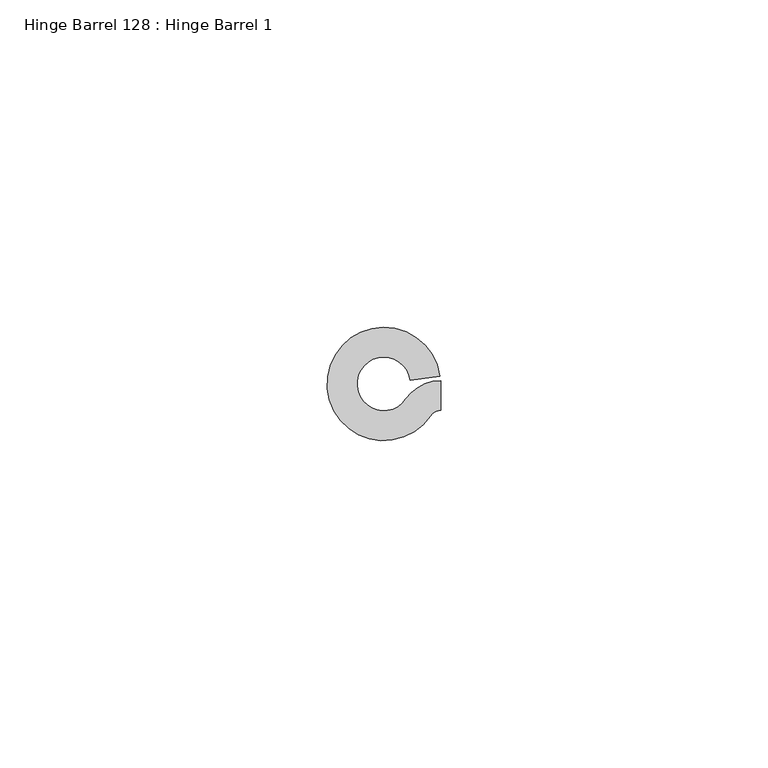
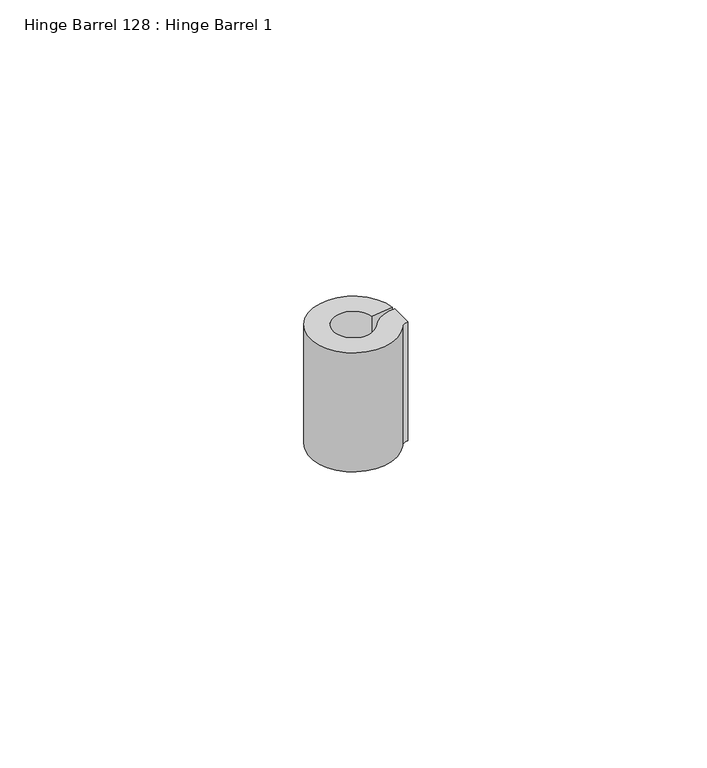
"""IFC4 building model written with IfcOpenShell, lengths in millimetres: proxy geometry, Hinge Barrel 128 : Hinge Barrel 1."""

from ifc_helpers import new_model, si_unit, point, frame, frame_2d, origin, place, context, project, spatial, polyline, circle_curve, trimmed, segment, composite_curve, outline, extrude, source, transform, mapped, element, save


def hinge_barrel_128_hinge_barrel_1_d11eb973(model_context):
    return source(origin(), model_context, "Body", "SweptSolid", [
        extrude(outline(composite_curve([segment(trimmed(circle_curve(frame_2d((587327.8245257, -536316.2443067)), 6.4044851), [point((587322.5194669, -536312.6563017))], [point((587327.8245257, -536309.8398216))], False, "CARTESIAN"), True, "CONTINUOUS"), segment(polyline([(587327.8245257, -536309.8398216), (587327.8245257, -536314.4038841)]), True, "CONTINUOUS"), segment(trimmed(circle_curve(frame_2d((587327.8245257, -536316.2443067)), 1.8404226), [point((587327.8245257, -536314.4038841))], [point((587326.3000393, -536315.2132409))], True, "CARTESIAN"), True, "CONTINUOUS"), segment(trimmed(circle_curve(frame_2d((587319.1320739, -536310.3652841)), 8.6534625), [point((587326.3000393, -536315.2132409))], [point((587327.7022899, -536309.1678654))], False, "CARTESIAN"), True, "CONTINUOUS"), segment(polyline([(587327.7022899, -536309.1678654), (587323.1821338, -536309.7994153)]), True, "CONTINUOUS"), segment(trimmed(circle_curve(frame_2d((587319.1320739, -536310.3652841)), 4.0894), [point((587323.1821338, -536309.7994153))], [point((587322.5194669, -536312.6563017))], True, "CARTESIAN"), True, "CONTINUOUS")], self_intersect=False)), frame((0.0, 0.0, 336.55), z_axis=(0.0, 0.0, 1.0), x_axis=(1.0, 0.0, 0.0)), (0.0, 0.0, 1.0), 25.4),
    ])


if __name__ == "__main__":
    model = new_model("IFC4")
    model_context = context("Model", 3, world=origin())
    ifc_project = project(units=[si_unit("LENGTHUNIT", "METRE", prefix="MILLI")], contexts=[model_context])
    site = spatial("IfcSite", under=ifc_project)
    building = spatial("IfcBuilding", under=site)
    placement = place(None, origin())
    hinge_barrel_128_hinge_barrel_1_shape = hinge_barrel_128_hinge_barrel_1_d11eb973(model_context)
    element("IfcBuildingElementProxy", 1, Name="Hinge Barrel 128 : Hinge Barrel 1", ObjectType="Hinge Barrel 128 : Hinge Barrel 1", at=placement, inside=building, context=model_context, shape_type="MappedRepresentation", body=[
        mapped(hinge_barrel_128_hinge_barrel_1_shape, transform((0.0, 0.0, 0.0), x_axis=(1.0, 0.0, 0.0), y_axis=(0.0, 1.0, 0.0), z_axis=(0.0, 0.0, 1.0))),
    ])
    save(model, "model.ifc")

# Revit data of these elements
# Element 1 (IfcBuildingElementProxy, "Hinge Barrel 128 : Hinge Barrel 1")
#   Materials on its faces: "6\"X6\" WELD-ON STL BUTT HINGE"
# Materials
#   "6\"X6\" WELD-ON STL BUTT HINGE": class "Metal", colour RGB 189 187 185, transparency 0, Description = "Carbon steel", Cost = 0
